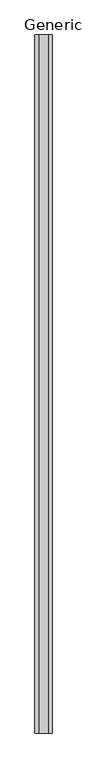
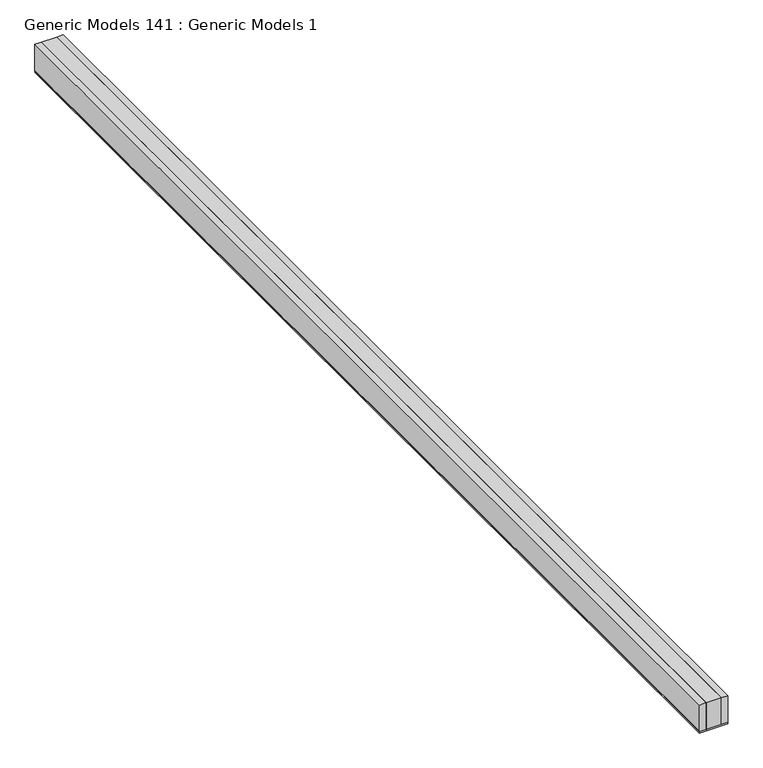
"""IFC4 building model written with IfcOpenShell, lengths in millimetres: proxy geometry, Generic Models 141 : Generic Models 1."""

from ifc_helpers import new_model, si_unit, point, frame, frame_2d, origin, place, context, project, spatial, polyline, circle_curve, trimmed, segment, composite_curve, outline, extrude, source, transform, mapped, element, save


def generic_models_141_generic_models_1_07cb97cc(model_context):
    return source(origin(), model_context, "Body", "SweptSolid", [
        extrude(outline(polyline([(-9801.3170959, 2393.3769662), (-9756.8670959, 2393.3769662), (-9756.8670959, -5493.3230338), (-9801.3170959, -5493.3230338), (-9801.3170959, 2393.3769662)])), frame((0.0, 0.0, 123149.5656204), z_axis=(0.0, 0.0, 1.0), x_axis=(1.0, 0.0, 0.0)), (0.0, 0.0, 1.0), 193.675),
        extrude(outline(composite_curve([segment(polyline([(123149.1687454, -9756.8670959), (123149.1687454, -9950.5420959)]), True, "CONTINUOUS"), segment(trimmed(circle_curve(frame_2d((123144.6046829, -9954.9570516)), 6.35), [point((123149.1687454, -9950.5420959))], [point((123140.0406204, -9950.5420959))], True, "CARTESIAN"), True, "CONTINUOUS"), segment(polyline([(123140.0406204, -9950.5420959), (123140.0406204, -9756.8670959)]), True, "CONTINUOUS"), segment(trimmed(circle_curve(frame_2d((123144.6046829, -9752.4521402)), 6.35), [point((123140.0406204, -9756.8670959))], [point((123149.1687454, -9756.8670959))], True, "CARTESIAN"), True, "CONTINUOUS")], self_intersect=False)), frame((0.0, -5493.3230338, 0.0), z_axis=(0.0, 1.0, 0.0), x_axis=(0.0, 0.0, 1.0)), (0.0, 0.0, 1.0), 7886.7),
        extrude(outline(polyline([(-9905.6952209, 2393.3769662), (-9801.7139709, 2393.3769662), (-9801.7139709, -5493.3230338), (-9905.6952209, -5493.3230338), (-9905.6952209, 2393.3769662)])), frame((0.0, 0.0, 123149.5656204), z_axis=(0.0, 0.0, 1.0), x_axis=(1.0, 0.0, 0.0)), (0.0, 0.0, 1.0), 193.675),
        extrude(outline(polyline([(-9950.5420959, 2393.3769662), (-9906.0920959, 2393.3769662), (-9906.0920959, -5493.3230338), (-9950.5420959, -5493.3230338), (-9950.5420959, 2393.3769662)])), frame((0.0, 0.0, 123149.5656204), z_axis=(0.0, 0.0, 1.0), x_axis=(1.0, 0.0, 0.0)), (0.0, 0.0, 1.0), 193.675),
    ])


if __name__ == "__main__":
    model = new_model("IFC4")
    model_context = context("Model", 3, world=origin())
    ifc_project = project(units=[si_unit("LENGTHUNIT", "METRE", prefix="MILLI")], contexts=[model_context])
    site = spatial("IfcSite", under=ifc_project)
    building = spatial("IfcBuilding", under=site)
    placement = place(None, origin())
    generic_models_141_generic_models_1_shape = generic_models_141_generic_models_1_07cb97cc(model_context)
    element("IfcBuildingElementProxy", 1, Name="Generic Models 141 : Generic Models 1", ObjectType="Generic Models 141 : Generic Models 1", at=placement, inside=building, context=model_context, shape_type="MappedRepresentation", body=[
        mapped(generic_models_141_generic_models_1_shape, transform((0.0, 0.0, 0.0), x_axis=(1.0, 0.0, 0.0), y_axis=(0.0, 1.0, 0.0), z_axis=(0.0, 0.0, 1.0))),
    ])
    save(model, "model.ifc")

# Revit data of these elements
# Element 1 (IfcBuildingElementProxy, "Generic Models 141 : Generic Models 1")
#   Materials on its faces: "_CONCRETE MASONRY UNITS - FILLED CORE - (SEE STRUCT. DWGS)"
# Materials
#   "_CONCRETE MASONRY UNITS - FILLED CORE - (SEE STRUCT. DWGS)": class "Generic", colour RGB 191 191 191, transparency 0, Cost = 0
